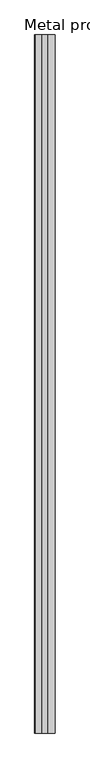
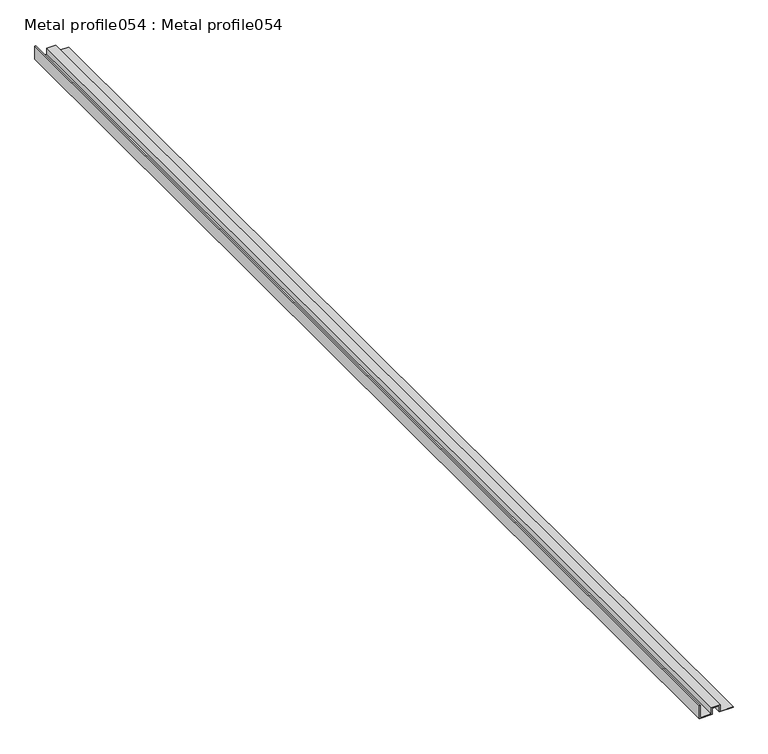
"""IFC4 building model written with IfcOpenShell, lengths in millimetres: proxy geometry, Metal profile054 : Metal profile054."""

from ifc_helpers import new_model, si_unit, frame, origin, place, context, project, spatial, polyline, outline, extrude, source, transform, mapped, element, save


def metal_profile054_metal_profile054_d53b2102(model_context):
    return source(origin(), model_context, "Body", "SweptSolid", [
        extrude(outline(polyline([(39543.8875708, -2790.7255764), (39543.8875708, -2768.5005764), (39555.3175708, -2768.5005764), (39555.3175708, -2755.8005764), (39543.8875708, -2755.8005764), (39543.8875708, -2732.0873925), (39545.1675708, -2732.0873925), (39545.1675708, -2754.5205764), (39556.5975708, -2754.5205764), (39556.5975708, -2769.7805764), (39545.1675708, -2769.7805764), (39545.1675708, -2789.4455764), (39567.6883323, -2789.4455764), (39567.6883323, -2790.7255764), (39543.8875708, -2790.7255764)])), frame((0.0, -1052.8906574, 0.0), z_axis=(0.0, 1.0, 0.0), x_axis=(0.0, 0.0, 1.0)), (0.0, 0.0, 1.0), 2000.0),
    ])


if __name__ == "__main__":
    model = new_model("IFC4")
    model_context = context("Model", 3, world=origin())
    ifc_project = project(units=[si_unit("LENGTHUNIT", "METRE", prefix="MILLI")], contexts=[model_context])
    site = spatial("IfcSite", under=ifc_project)
    building = spatial("IfcBuilding", under=site)
    placement = place(None, origin())
    metal_profile054_metal_profile054_shape = metal_profile054_metal_profile054_d53b2102(model_context)
    element("IfcBuildingElementProxy", 1, Name="Metal profile054 : Metal profile054", ObjectType="Metal profile054 : Metal profile054", at=placement, inside=building, context=model_context, shape_type="MappedRepresentation", body=[
        mapped(metal_profile054_metal_profile054_shape, transform((0.0, 0.0, 0.0), x_axis=(1.0, 0.0, 0.0), y_axis=(0.0, 1.0, 0.0), z_axis=(0.0, 0.0, 1.0))),
    ])
    save(model, "model.ifc")

# Revit data of these elements
# Type "Metal profile054 : Metal profile054"
#   NameOverride = "Metal profile054"
# Element 1 (IfcBuildingElementProxy, "Metal profile054 : Metal profile054")
#   Materials on its faces: "16 GA. COPPER SOFFIT DRIP SCREED"
# Materials
#   "16 GA. COPPER SOFFIT DRIP SCREED": class "Unassigned", colour RGB 255 217 0, transparency 0
